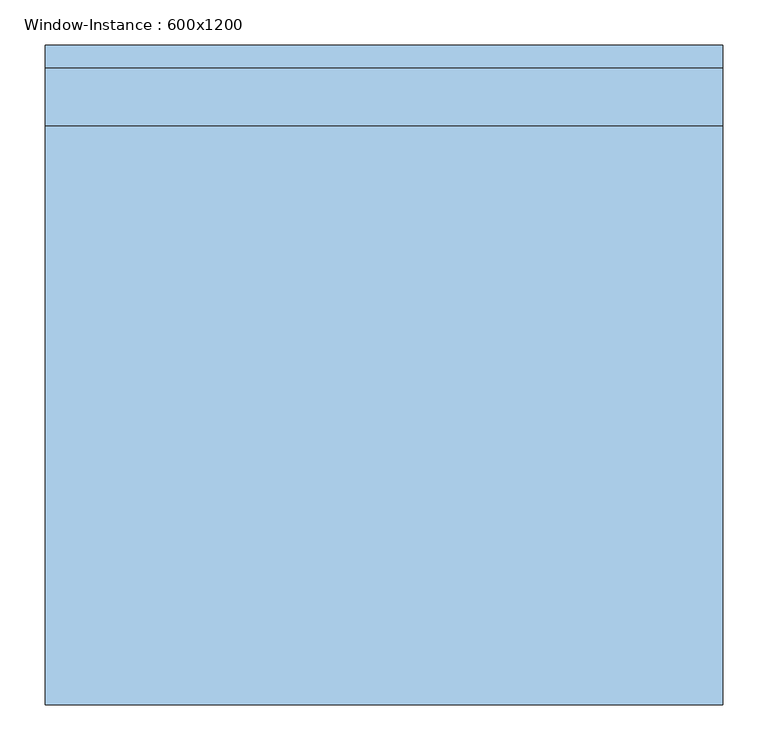
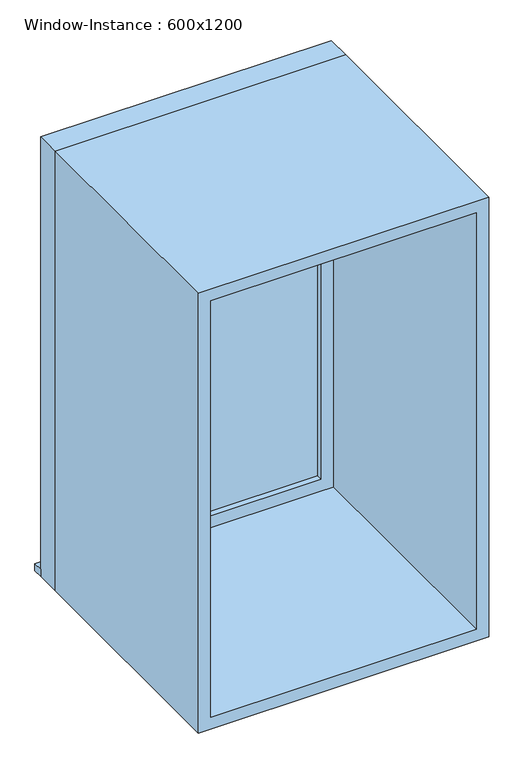
"""IFC4 building model written with IfcOpenShell, lengths in millimetres: window geometry, Window-Instance : 600x1200."""

from ifc_helpers import new_model, si_unit, frame, origin, place, context, project, spatial, polyline, outline, extrude, source, transform, mapped, element, save


def window_instance_600x1200_74739665(model_context):
    return source(origin(), model_context, "Body", "SweptSolid", [
        extrude(outline(polyline([(-413.1, 377.9), (336.9, 377.9), (336.9, 352.5), (-413.1, 352.5), (-413.1, 377.9)])), frame((0.0, 0.0, 900.0), z_axis=(0.0, 0.0, 1.0), x_axis=(1.0, 0.0, 0.0)), (0.0, 0.0, 1.0), 19.05),
        extrude(outline(polyline([(273.4, 303.925), (-349.6, 303.925), (-349.6, 316.625), (273.4, 316.625), (273.4, 303.925)])), frame((0.0, 0.0, 963.5), z_axis=(0.0, 0.0, 1.0), x_axis=(1.0, 0.0, 0.0)), (0.0, 0.0, 1.0), 1073.0),
        extrude(outline(polyline([(2080.95, -394.05), (919.05, -394.05), (919.05, 317.85), (2080.95, 317.85), (2080.95, -394.05)]), holes=[polyline([(2036.5, -349.6), (2036.5, 273.4), (963.5, 273.4), (963.5, -349.6), (2036.5, -349.6)])]), frame((0.0, 288.05, 0.0), z_axis=(0.0, 1.0, 0.0), x_axis=(0.0, 0.0, 1.0)), (0.0, 0.0, 1.0), 44.45),
        extrude(outline(polyline([(2100.0, -413.1), (900.0, -413.1), (900.0, 336.9), (2100.0, 336.9), (2100.0, -413.1)]), holes=[polyline([(2068.25, -381.35), (2068.25, 305.15), (931.75, 305.15), (931.75, -381.35), (2068.25, -381.35)])]), frame((0.0, -352.5, 0.0), z_axis=(0.0, 1.0, 0.0), x_axis=(0.0, 0.0, 1.0)), (0.0, 0.0, 1.0), 640.55),
        extrude(outline(polyline([(2100.0, 336.9), (2100.0, -413.1), (900.0, -413.1), (900.0, 336.9), (2100.0, 336.9)]), holes=[polyline([(2080.95, 317.85), (919.05, 317.85), (919.05, -394.05), (2080.95, -394.05), (2080.95, 317.85)])]), frame((0.0, 288.05, 0.0), z_axis=(0.0, 1.0, 0.0), x_axis=(0.0, 0.0, 1.0)), (0.0, 0.0, 1.0), 64.45),
    ])


if __name__ == "__main__":
    model = new_model("IFC4")
    model_context = context("Model", 3, world=origin())
    ifc_project = project(units=[si_unit("LENGTHUNIT", "METRE", prefix="MILLI")], contexts=[model_context])
    site = spatial("IfcSite", under=ifc_project)
    building = spatial("IfcBuilding", under=site)
    placement = place(None, origin())
    window_instance_600x1200_shape = window_instance_600x1200_74739665(model_context)
    element("IfcWindow", 1, ObjectType="Window-Instance : 600x1200", at=placement, inside=building, context=model_context, shape_type="MappedRepresentation", body=[
        mapped(window_instance_600x1200_shape, transform((0.0, 0.0, 0.0), x_axis=(1.0, 0.0, 0.0), y_axis=(0.0, 1.0, 0.0), z_axis=(0.0, 0.0, 1.0))),
    ])
    save(model, "model.ifc")

# Revit data of these elements
# Type "Window-Instance : 600x1200"
#   Type Mark = "7"
#   Construction Type Id = "GSP4R"
#   Assembly Code = "B2020100"
#   Analytic Construction = "1/8 in Pilkington single glazing"
#   Visual Light Transmittance = 0.9
#   Thermal Resistance (R) = 0.149095 (m²·K)/W
#   Solar Heat Gain Coefficient = 0.86
#   Heat Transfer Coefficient (U) = 6.70716 W/(m²·K)
#   Height [instance default] = 1200 mm
#   Default Sill Height = 900 mm
#   Width [instance default] = 600 mm
#   Window Inset = 20 mm
#   Glass Pane Material = WW-EC-GL-Storefront
#   Sash Material = WW-EC-RGB-White
#   Wall Closure = (empty or 0)
# Element 1 (IfcWindow, "Window-Instance : 600x1200")
#   Width = 750 mm
#   Materials on its faces: "WW-EC-RGB-White", "WW-EC-GL-Storefront"
# Materials
#   "WW-EC-GL-Storefront": class "Glass", colour RGB 236 240 239, transparency 0.85, Description = "Storefront Glass", Cost = 0
#   "WW-EC-RGB-White": class "Generic", colour RGB 255 255 255, transparency 0, Comments = "If region requests off-white, swith asset color to RGB 231-228-220", Description = "Generic Color", Cost = 0
